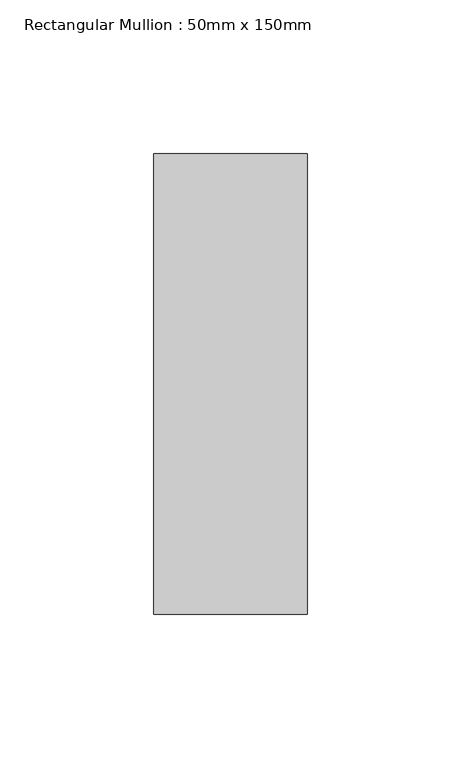
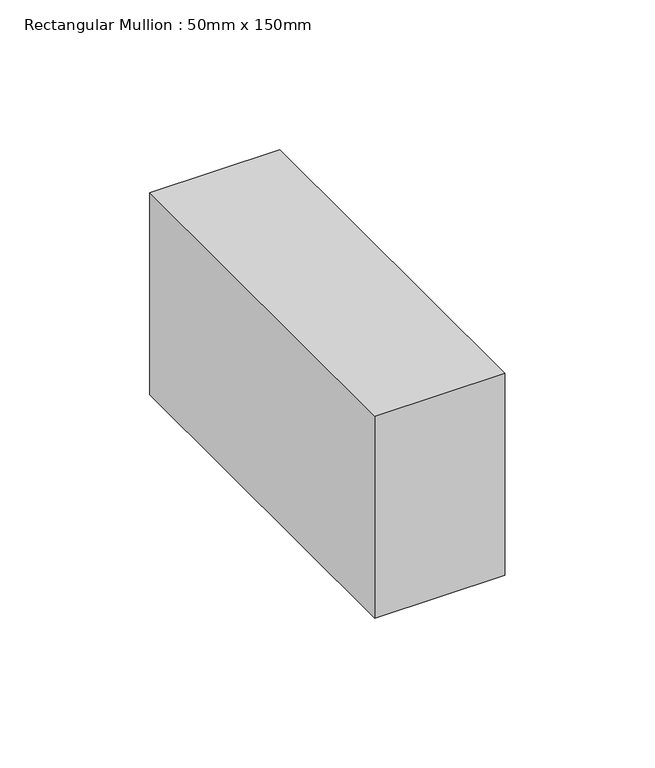
"""IFC4 building model written with IfcOpenShell, lengths in millimetres: member geometry, Rectangular Mullion : 50mm x 150mm."""

from ifc_helpers import new_model, si_unit, frame, origin, place, context, project, spatial, polyline, outline, extrude, source, transform, mapped, element, save


def rectangular_mullion_50mm_x_150mm_8699f243(model_context):
    return source(origin(), model_context, "Body", "SweptSolid", [
        extrude(outline(polyline([(0.0, 75.0), (0.0, -75.0), (-50.0, -75.0), (-50.0, 75.0), (0.0, 75.0)])), frame((0.0, 0.0, -82.0909088), z_axis=(0.0, 0.0, 1.0), x_axis=(1.0, 0.0, 0.0)), (0.0, 0.0, 1.0), 82.0909088),
    ])


if __name__ == "__main__":
    model = new_model("IFC4")
    model_context = context("Model", 3, world=origin())
    ifc_project = project(units=[si_unit("LENGTHUNIT", "METRE", prefix="MILLI")], contexts=[model_context])
    site = spatial("IfcSite", under=ifc_project)
    building = spatial("IfcBuilding", under=site)
    placement = place(None, origin())
    rectangular_mullion_50mm_x_150mm_shape = rectangular_mullion_50mm_x_150mm_8699f243(model_context)
    element("IfcMember", 1, ObjectType="Rectangular Mullion : 50mm x 150mm", at=placement, inside=building, context=model_context, shape_type="MappedRepresentation", body=[
        mapped(rectangular_mullion_50mm_x_150mm_shape, transform((0.0, 0.0, 0.0), x_axis=(1.0, 0.0, 0.0), y_axis=(0.0, 1.0, 0.0), z_axis=(0.0, 0.0, 1.0))),
    ])
    save(model, "model.ifc")

# Revit data of these elements
# Type "Rectangular Mullion : 50mm x 150mm"
#   built-in parameter 1007304 = 0.492126 (stored number, unit not read)
#   built-in parameter 1007301 = 0.082021 (stored number, unit not read)
#   built-in parameter 1007300 = 0.082021 (stored number, unit not read)
# Element 1 (IfcMember, "Rectangular Mullion : 50mm x 150mm")
#   Materials on its faces: "Aluminum"
# Materials
#   "Aluminum": class "Metal", colour RGB 244 244 244, transparency 0, Description = "Aluminum 6061", Cost = 0
